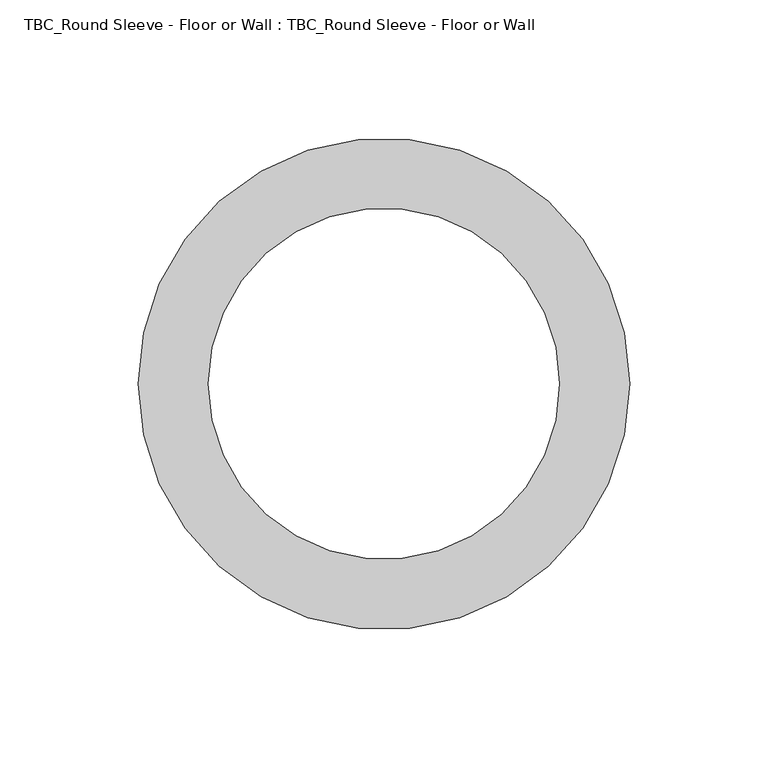
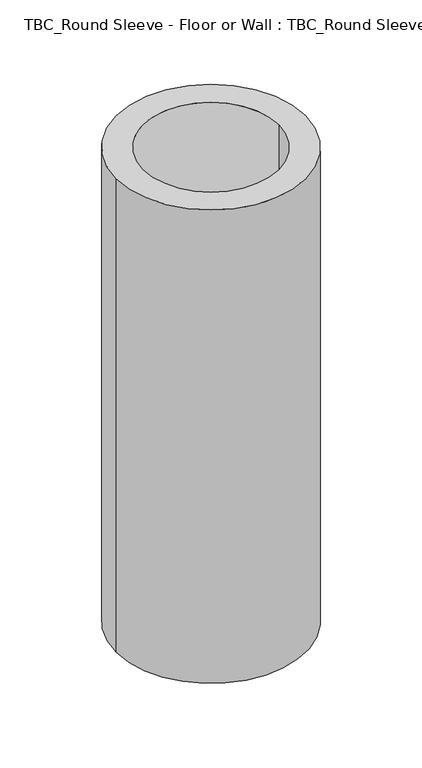
"""IFC4 building model written with IfcOpenShell, lengths in millimetres: proxy geometry, TBC_Round Sleeve - Floor or Wall : TBC_Round Sleeve - Floor or Wall."""

from ifc_helpers import new_model, si_unit, point, frame, origin, origin_2d, place, context, project, spatial, circle_curve, trimmed, segment, composite_curve, outline, extrude, source, transform, mapped, element, save


def tbc_round_sleeve_floor_or_wall_tbc_round_sleeve_floor_or_275ba5eb(model_context):
    return source(origin(), model_context, "Body", "SweptSolid", [
        extrude(outline(composite_curve([segment(trimmed(circle_curve(origin_2d(), 88.9), [point((-88.9, 0.0))], [point((88.9, 0.0))], False, "CARTESIAN"), True, "CONTINUOUS"), segment(trimmed(circle_curve(origin_2d(), 88.9), [point((88.9, 0.0))], [point((-88.9, 0.0))], False, "CARTESIAN"), True, "CONTINUOUS")], self_intersect=False), holes=[composite_curve([segment(trimmed(circle_curve(origin_2d(), 63.5), [point((-63.5, 0.0))], [point((63.5, 0.0))], True, "CARTESIAN"), True, "CONTINUOUS"), segment(trimmed(circle_curve(origin_2d(), 63.5), [point((63.5, 0.0))], [point((-63.5, 0.0))], True, "CARTESIAN"), True, "CONTINUOUS")], self_intersect=False)]), frame((0.0, 0.0, -469.9), z_axis=(0.0, 0.0, 1.0), x_axis=(1.0, 0.0, 0.0)), (0.0, 0.0, 1.0), 469.9),
    ])


if __name__ == "__main__":
    model = new_model("IFC4")
    model_context = context("Model", 3, world=origin())
    ifc_project = project(units=[si_unit("LENGTHUNIT", "METRE", prefix="MILLI")], contexts=[model_context])
    site = spatial("IfcSite", under=ifc_project)
    building = spatial("IfcBuilding", under=site)
    placement = place(None, origin())
    tbc_round_sleeve_floor_or_wall_tbc_round_sleeve_floor_or_shape = tbc_round_sleeve_floor_or_wall_tbc_round_sleeve_floor_or_275ba5eb(model_context)
    element("IfcBuildingElementProxy", 1, Name="TBC_Round Sleeve - Floor or Wall : TBC_Round Sleeve - Floor or Wall", ObjectType="TBC_Round Sleeve - Floor or Wall : TBC_Round Sleeve - Floor or Wall", at=placement, inside=building, context=model_context, shape_type="MappedRepresentation", body=[
        mapped(tbc_round_sleeve_floor_or_wall_tbc_round_sleeve_floor_or_shape, transform((0.0, 0.0, 0.0), x_axis=(1.0, 0.0, 0.0), y_axis=(0.0, 1.0, 0.0), z_axis=(0.0, 0.0, 1.0))),
    ])
    save(model, "model.ifc")

# Revit data of these elements
# Type "TBC_Round Sleeve - Floor or Wall : TBC_Round Sleeve - Floor or Wall"
#   Tag Dimension [instance default] = ""
#   MEP Type [instance default] = ""
#   MEP Element [instance default] = ""
#   MEP Category [instance default] = ""
#   Host Element Type [instance default] = ""
#   Host Element Id [instance default] = ""
#   Host Element Category [instance default] = ""
#   Control Line Y [instance default] = ""
#   Control Line X [instance default] = ""
#   Sleeve Radius [instance default] = 1' - 0"
#   Sleeve Edge [instance default] = 1' - 2"
#   Sleeve Depth [instance default] = 3' - 0"
#   Distance Y [instance default] = 0' - 0"
#   Distance X [instance default] = 0' - 0"
#   Default Elevation = 0
# Element 1 (IfcBuildingElementProxy, "TBC_Round Sleeve - Floor or Wall : TBC_Round Sleeve - Floor or Wall")
#   MEP Type = "PLG-ST"
#   MEP Element = "828279"
#   MEP Category = "Pipe"
#   Host Element Type = "Roof Plank-Sleeves"
#   Host Element Id = "1525183"
#   Host Element Category = "Floors"
#   Sleeve Radius = 0' - 5"
#   Sleeve Edge = 0' - 7"
#   Sleeve Depth = 1' - 6 1/2"
